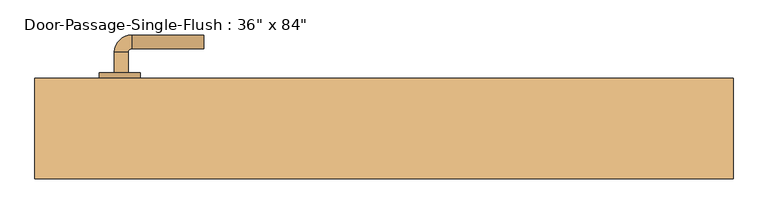
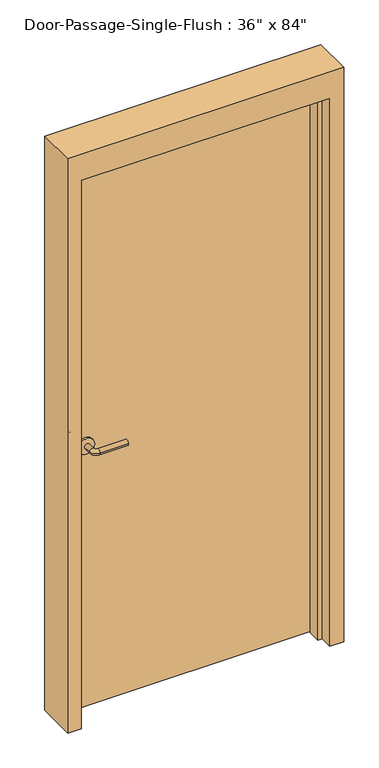
"""IFC4 building model written with IfcOpenShell, lengths in millimetres: door geometry."""

from ifc_helpers import new_model, si_unit, point, frame, frame_2d, origin, origin_with_axes, place, context, project, spatial, polyline, circle_curve, ellipse_curve, trimmed, segment, composite_curve, outline, extrude, faceted_brep, source, transform, mapped, element, save
from ifc_brep_helpers import plane_surface, cylinder_surface, revolved_surface, advanced_brep


def door_12021f76(model_context):
    return source(origin(), model_context, "Body", "SolidModel", [
        advanced_brep(
        [(-392.190625, -9.5875, 1016.0), (-372.190625, -9.5875, 1016.0), (-372.190625, -39.5875, 1016.0), (-392.190625, -39.5875, 1016.0), (-367.190625, -44.5875, 1016.0), (-367.190625, -64.5875, 1016.0), (-262.190625, -64.5875, 1016.0), (-262.190625, -44.5875, 1016.0)],
        [
            (0, 1, circle_curve(frame((-382.190625, -9.5875, 1016.0), z_axis=(0.0, 1.0, 0.0), x_axis=(1.0, 0.0, 0.0)), 10.0)),
            (1, 0, circle_curve(frame((-382.190625, -9.5875, 1016.0), z_axis=(0.0, 1.0, 0.0), x_axis=(1.0, 0.0, 0.0)), 10.0)),
            (1, 2),
            (2, 3, circle_curve(frame((-382.190625, -39.5875, 1016.0), z_axis=(0.0, 1.0, 0.0), x_axis=(1.0, 0.0, 0.0)), 10.0)),
            (3, 0),
            (3, 2, circle_curve(frame((-382.190625, -39.5875, 1016.0), z_axis=(0.0, 1.0, 0.0), x_axis=(1.0, 0.0, 0.0)), 10.0)),
            (4, 5, circle_curve(frame((-367.190625, -54.5875, 1016.0), z_axis=(-1.0, 0.0, 0.0), x_axis=(0.0, 1.0, 0.0)), 10.0)),
            (5, 3, circle_curve(frame((-367.190625, -39.5875, 1016.0), z_axis=(0.0, 0.0, -1.0), x_axis=(-1.0, 0.0, 0.0)), 25.0)),
            (2, 4, circle_curve(frame((-367.190625, -39.5875, 1016.0), z_axis=(0.0, 0.0, 1.0), x_axis=(-1.0, 0.0, 0.0)), 5.0)),
            (5, 4, circle_curve(frame((-367.190625, -54.5875, 1016.0), z_axis=(-1.0, 0.0, 0.0), x_axis=(0.0, 1.0, 0.0)), 10.0)),
            (6, 7, circle_curve(frame((-262.190625, -54.5875, 1016.0), z_axis=(1.0, 0.0, 0.0), x_axis=(0.0, 1.0, 0.0)), 10.0)),
            (7, 6, circle_curve(frame((-262.190625, -54.5875, 1016.0), z_axis=(1.0, 0.0, 0.0), x_axis=(0.0, 1.0, 0.0)), 10.0)),
            (4, 7),
            (6, 5),
        ],
        [
            plane_surface(frame((-382.190625, -9.5875, 1016.0), z_axis=(0.0, 1.0, 0.0), x_axis=(0.0, 0.0, 1.0))),
            cylinder_surface(frame((-382.190625, -9.5875, 1016.0), z_axis=(0.0, 1.0, 0.0), x_axis=(1.0, 0.0, 0.0)), 10.0),
            revolved_surface(trimmed(ellipse_curve(frame((-382.190625, -39.5875, 1016.0), z_axis=(0.0, -1.0, 0.0), x_axis=(1.0, 0.0, 0.0)), 10.0, 10.0), [point((-392.190625, -39.5875, 1016.0))], [point((-372.190625, -39.5875, 1016.0))], True, "CARTESIAN"), (-367.190625, -39.5875, 1016.0), (0.0, 0.0, -1.0)),
            revolved_surface(trimmed(ellipse_curve(frame((-382.190625, -39.5875, 1016.0), z_axis=(0.0, -1.0, 0.0), x_axis=(1.0, 0.0, 0.0)), 10.0, 10.0), [point((-372.190625, -39.5875, 1016.0))], [point((-392.190625, -39.5875, 1016.0))], True, "CARTESIAN"), (-367.190625, -39.5875, 1016.0), (0.0, 0.0, -1.0)),
            plane_surface(frame((-262.190625, -54.5875, 1016.0), z_axis=(1.0, 0.0, 0.0), x_axis=(0.0, 0.0, 1.0))),
            cylinder_surface(frame((-367.190625, -54.5875, 1016.0), z_axis=(-1.0, 0.0, 0.0), x_axis=(0.0, 1.0, 0.0)), 10.0),
        ],
        [
            (0, [[1, 2]]),
            (1, [[3, 4, 5, -2]]),
            (1, [[-5, 6, -3, -1]]),
            (2, [[7, 8, -4, 9]]),
            (3, [[10, -9, -6, -8]]),
            (4, [[11, 12]]),
            (5, [[13, -11, 14, -7]]),
            (5, [[-14, -12, -13, -10]]),
        ],
    ),
        extrude(outline(composite_curve([segment(trimmed(circle_curve(frame_2d((1016.0, -384.690625)), 30.0), [point((1016.0, -414.690625))], [point((1016.0, -354.690625))], False, "CARTESIAN"), True, "CONTINUOUS"), segment(trimmed(circle_curve(frame_2d((1016.0, -384.690625)), 30.0), [point((1016.0, -354.690625))], [point((1016.0, -414.690625))], False, "CARTESIAN"), True, "CONTINUOUS")], self_intersect=False)), frame((0.0, -9.5875, 0.0), z_axis=(0.0, 1.0, 0.0), x_axis=(0.0, 0.0, 1.0)), (0.0, 0.0, 1.0), 8.0),
        advanced_brep(
        [(-392.190625, 50.8625, 1016.0), (-372.190625, 50.8625, 1016.0), (-392.190625, 80.8625, 1016.0), (-372.190625, 80.8625, 1016.0), (-367.190625, 85.8625, 1016.0), (-367.190625, 105.8625, 1016.0), (-262.190625, 105.8625, 1016.0), (-262.190625, 85.8625, 1016.0)],
        [
            (0, 1, circle_curve(frame((-382.190625, 50.8625, 1016.0), z_axis=(0.0, -1.0, 0.0), x_axis=(1.0, 0.0, 0.0)), 10.0)),
            (1, 0, circle_curve(frame((-382.190625, 50.8625, 1016.0), z_axis=(0.0, -1.0, 0.0), x_axis=(1.0, 0.0, 0.0)), 10.0)),
            (0, 2),
            (2, 3, circle_curve(frame((-382.190625, 80.8625, 1016.0), z_axis=(0.0, -1.0, 0.0), x_axis=(1.0, 0.0, 0.0)), 10.0)),
            (3, 1),
            (3, 2, circle_curve(frame((-382.190625, 80.8625, 1016.0), z_axis=(0.0, -1.0, 0.0), x_axis=(1.0, 0.0, 0.0)), 10.0)),
            (4, 3, circle_curve(frame((-367.190625, 80.8625, 1016.0), z_axis=(0.0, 0.0, 1.0), x_axis=(-1.0, 0.0, 0.0)), 5.0)),
            (2, 5, circle_curve(frame((-367.190625, 80.8625, 1016.0), z_axis=(0.0, 0.0, -1.0), x_axis=(-1.0, 0.0, 0.0)), 25.0)),
            (5, 4, circle_curve(frame((-367.190625, 95.8625, 1016.0), z_axis=(-1.0, 0.0, 0.0), x_axis=(0.0, -1.0, 0.0)), 10.0)),
            (4, 5, circle_curve(frame((-367.190625, 95.8625, 1016.0), z_axis=(-1.0, 0.0, 0.0), x_axis=(0.0, -1.0, 0.0)), 10.0)),
            (6, 7, circle_curve(frame((-262.190625, 95.8625, 1016.0), z_axis=(1.0, 0.0, 0.0), x_axis=(0.0, -1.0, 0.0)), 10.0)),
            (7, 6, circle_curve(frame((-262.190625, 95.8625, 1016.0), z_axis=(1.0, 0.0, 0.0), x_axis=(0.0, -1.0, 0.0)), 10.0)),
            (5, 6),
            (7, 4),
        ],
        [
            plane_surface(frame((-382.190625, 50.8625, 1016.0), z_axis=(0.0, -1.0, 0.0), x_axis=(0.0, 0.0, 1.0))),
            cylinder_surface(frame((-382.190625, 50.8625, 1016.0), z_axis=(0.0, -1.0, 0.0), x_axis=(1.0, 0.0, 0.0)), 10.0),
            revolved_surface(trimmed(ellipse_curve(frame((-382.190625, 80.8625, 1016.0), z_axis=(0.0, -1.0, 0.0), x_axis=(1.0, 0.0, 0.0)), 10.0, 10.0), [point((-392.190625, 80.8625, 1016.0))], [point((-372.190625, 80.8625, 1016.0))], True, "CARTESIAN"), (-367.190625, 80.8625, 1016.0), (0.0, 0.0, -1.0)),
            revolved_surface(trimmed(ellipse_curve(frame((-382.190625, 80.8625, 1016.0), z_axis=(0.0, -1.0, 0.0), x_axis=(1.0, 0.0, 0.0)), 10.0, 10.0), [point((-372.190625, 80.8625, 1016.0))], [point((-392.190625, 80.8625, 1016.0))], True, "CARTESIAN"), (-367.190625, 80.8625, 1016.0), (0.0, 0.0, -1.0)),
            plane_surface(frame((-262.190625, 95.8625, 1016.0), z_axis=(1.0, 0.0, 0.0), x_axis=(0.0, 0.0, 1.0))),
            cylinder_surface(frame((-367.190625, 95.8625, 1016.0), z_axis=(-1.0, 0.0, 0.0), x_axis=(0.0, -1.0, 0.0)), 10.0),
        ],
        [
            (0, [[1, 2]]),
            (1, [[-1, 3, 4, 5]]),
            (1, [[-2, -5, 6, -3]]),
            (2, [[7, -4, 8, 9]]),
            (3, [[-8, -6, -7, 10]]),
            (4, [[11, 12]]),
            (5, [[-9, 13, -12, 14]]),
            (5, [[-10, -14, -11, -13]]),
        ],
    ),
        extrude(outline(composite_curve([segment(trimmed(circle_curve(frame_2d((1016.0, -384.690625)), 30.0), [point((1016.0, -414.690625))], [point((1016.0, -354.690625))], False, "CARTESIAN"), True, "CONTINUOUS"), segment(trimmed(circle_curve(frame_2d((1016.0, -384.690625)), 30.0), [point((1016.0, -354.690625))], [point((1016.0, -414.690625))], False, "CARTESIAN"), True, "CONTINUOUS")], self_intersect=False)), frame((0.0, 42.8625, 0.0), z_axis=(0.0, 1.0, 0.0), x_axis=(0.0, 0.0, 1.0)), (0.0, 0.0, 1.0), 8.0),
        faceted_brep([(457.2, -6.35, 0.0), (457.2, 42.8625, 0.0), (508.0, 42.8625, 0.0), (508.0, -103.1875, 0.0), (457.2, -103.1875, 0.0), (457.2, -53.975, 0.0), (441.325, -53.975, 0.0), (441.325, -6.35, 0.0), (457.2, -6.35, 2133.6), (457.2, 42.8625, 2133.6), (-457.2, 42.8625, 2133.6), (-457.2, 42.8625, 0.0), (-508.0, 42.8625, 0.0), (-508.0, 42.8625, 2235.2), (508.0, 42.8625, 2235.2), (508.0, -103.1875, 2235.2), (-508.0, -103.1875, 2235.2), (-508.0, -103.1875, 0.0), (-457.2, -103.1875, 0.0), (-457.2, -103.1875, 2133.6), (457.2, -103.1875, 2133.6), (457.2, -53.975, 2133.6), (-457.2, -53.975, 2133.6), (-457.2, -53.975, 0.0), (-441.325, -53.975, 0.0), (-441.325, -53.975, 2117.725), (441.325, -53.975, 2117.725), (441.325, -6.35, 2117.725), (-441.325, -6.35, 2117.725), (-441.325, -6.35, 0.0), (-457.2, -6.35, 0.0), (-457.2, -6.35, 2133.6)], [[[0, 1, 2, 3, 4, 5, 6, 7]], [[1, 0, 8, 9]], [[2, 1, 9, 10, 11, 12, 13, 14]], [[3, 2, 14, 15]], [[4, 3, 15, 16, 17, 18, 19, 20]], [[5, 4, 20, 21]], [[6, 5, 21, 22, 23, 24, 25, 26]], [[7, 6, 26, 27]], [[0, 7, 27, 28, 29, 30, 31, 8]], [[9, 8, 31, 10]], [[20, 19, 22, 21]], [[26, 25, 28, 27]], [[12, 11, 30, 29, 24, 23, 18, 17]], [[11, 10, 31, 30]], [[13, 12, 17, 16]], [[19, 18, 23, 22]], [[25, 24, 29, 28]], [[15, 14, 13, 16]]]),
        extrude(outline(polyline([(457.2, -1.5875), (-457.2, -1.5875), (-457.2, 42.8625), (457.2, 42.8625), (457.2, -1.5875)])), origin_with_axes(), (0.0, 0.0, 1.0), 2133.6),
    ])


if __name__ == "__main__":
    model = new_model("IFC4")
    model_context = context("Model", 3, world=origin())
    ifc_project = project(units=[si_unit("LENGTHUNIT", "METRE", prefix="MILLI")], contexts=[model_context])
    site = spatial("IfcSite", under=ifc_project)
    building = spatial("IfcBuilding", under=site)
    placement = place(None, origin())
    door_shape = door_12021f76(model_context)
    element("IfcDoor", 1, ObjectType="Door-Passage-Single-Flush : 36\" x 84\"", at=placement, inside=building, context=model_context, shape_type="MappedRepresentation", body=[
        mapped(door_shape, transform((0.0, 0.0, 0.0), x_axis=(1.0, 0.0, 0.0), y_axis=(0.0, 1.0, 0.0), z_axis=(0.0, 0.0, 1.0))),
    ])
    save(model, "model.ifc")

# Revit data of these elements
# Type "Door-Passage-Single-Flush : 36\" x 84\""
#   Type Mark = "35"
#   Assembly Code = "B2030200"
#   Analytic Construction = "Wooden"
#   Thickness = 0' - 1 3/4"
#   Thermal Resistance (R) = 2.5876 (h·ft²·°F)/BTU
#   Swing Angle [instance default] = 90.00°
#   Strike Height = 3' - 4"
#   Rough Width [instance default] = 3' - 4"
#   Rough Height [instance default] = 7' - 4"
#   MF Opening Height [instance default] = 0' - 4"
#   MF Opening Width [instance default] = 0' - 4"
#   Inset Calculate [instance default] = 0' - 4"
#   Masonry Inset [instance default] = 0' - 1"
#   Height = 7' - 0"
#   Width = 3' - 0"
#   Heat Transfer Coefficient (U) = 0.3865 BTU/(h·ft²·°F)
#   Masonry Frame Depth = 0' - 5 3/4"
#   Masonry Frame [instance default] = yes
#   Function = 1
#   Dry Wall Frame [instance default] = no
#   Panel Material = Wood - Birch
#   Frame Material = Metal - Paint Finish - Grey
#   Door Handle Material = Aluminum
#   Visual Light Transmittance = 0
#   Solar Heat Gain Coefficient = 0
#   Wall Closure = (empty or 0)
# Element 1 (IfcDoor, "Door-Passage-Single-Flush : 36\" x 84\"")
#   Materials on its faces: "Aluminum", "Metal - Paint Finish - Grey", "Wood - Birch"
# Materials
#   "Wood - Birch": class "Wood", colour RGB 166 116 52, transparency 0, Cost = 0
#   "Metal - Paint Finish - Grey": class "Paint", colour RGB 104 104 104, transparency 0, Cost = 0
#   "Aluminum": class "Metal", colour RGB 247 247 247, transparency 0, Description = "Aluminum 6061", Cost = 0
